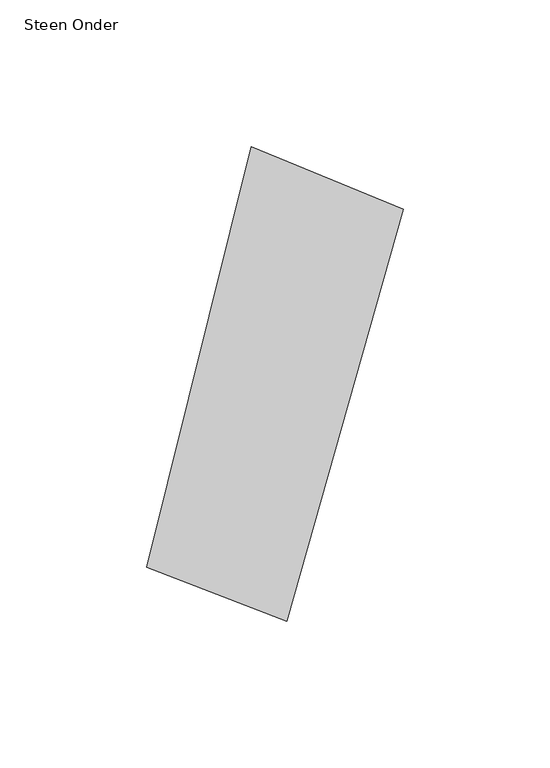
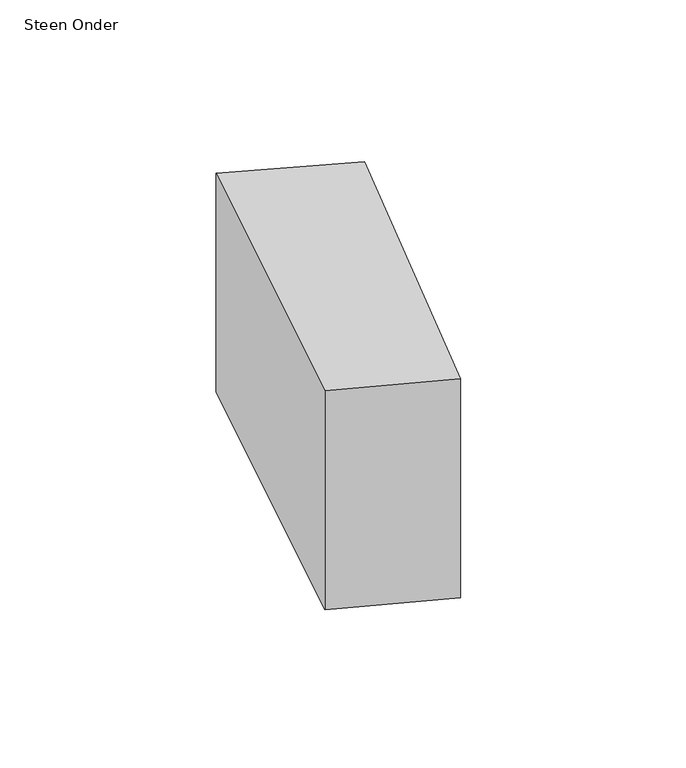
"""IFC4 building model written with IfcOpenShell, lengths in millimetres: proxy geometry, 00_GMA_steen_versie_4 : Steen Onder."""

from ifc_helpers import new_model, si_unit, origin, origin_with_axes, place, context, project, spatial, polyline, outline, extrude, source, transform, mapped, element, save


def steen_onder_4b1be589(model_context):
    return source(origin(), model_context, "Body", "SweptSolid", [
        extrude(outline(polyline([(120.1245435, 138.4089069), (80.3719859, -2.2262956), (32.5463602, 16.3140928), (68.2783004, 159.7130973), (120.1245435, 138.4089069)])), origin_with_axes(), (0.0, 0.0, 1.0), 100.0),
    ])


if __name__ == "__main__":
    model = new_model("IFC4")
    model_context = context("Model", 3, world=origin())
    ifc_project = project(units=[si_unit("LENGTHUNIT", "METRE", prefix="MILLI")], contexts=[model_context])
    site = spatial("IfcSite", under=ifc_project)
    building = spatial("IfcBuilding", under=site)
    placement = place(None, origin())
    steen_onder_shape = steen_onder_4b1be589(model_context)
    element("IfcBuildingElementProxy", 1, Name="00_GMA_steen_versie_4 : Steen Onder", ObjectType="00_GMA_steen_versie_4 : Steen Onder", at=placement, inside=building, context=model_context, shape_type="MappedRepresentation", body=[
        mapped(steen_onder_shape, transform((0.0, 0.0, 0.0), x_axis=(1.0, 0.0, 0.0), y_axis=(0.0, 1.0, 0.0), z_axis=(0.0, 0.0, 1.0))),
    ])
    save(model, "model.ifc")

# Revit data of these elements
# Type "00_GMA_steen_versie_4 : Steen Onder"
#   StootVoegHalfBoven [instance default] = 5 mm
#   StootVoegHalf [instance default] = 5 mm
#   StootVoegBreedteOnder = 10 mm
#   StootVoegBreedteBoven = 10 mm
#   Steendikte = 100 mm
#   LintVoegOnderHalf = 0 mm
#   LintVoegOnder = 0 mm
#   LintVoegBovenHalf = 5 mm
#   LintVoegBoven = 10 mm
#   materiaal = none
#   MateriaalVoeg = none
#   Default Elevation = 0
